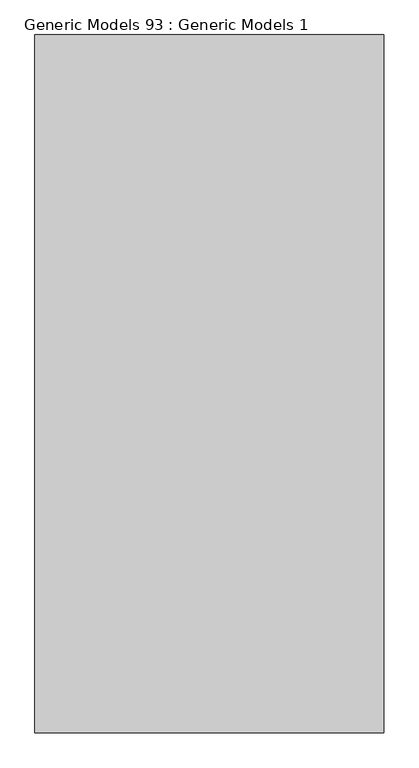
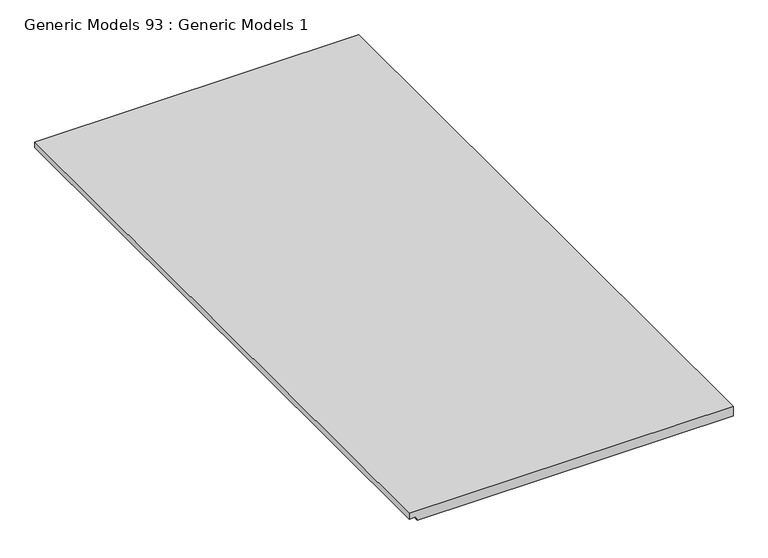
"""IFC4 building model written with IfcOpenShell, lengths in millimetres: proxy geometry, Generic Models 93 : Generic Models 1."""

from ifc_helpers import new_model, si_unit, frame, origin, place, context, project, spatial, polyline, outline, extrude, source, transform, mapped, element, save


def generic_models_93_generic_models_1_4e4062ca(model_context):
    return source(origin(), model_context, "Body", "SweptSolid", [
        extrude(outline(polyline([(2281.1808399, 49813.3451407), (2270.0683399, 49813.3451407), (2270.0683399, 49826.0451407), (2262.1308399, 49828.9341545), (2262.1308399, 50422.9451407), (2281.1808399, 50422.9451407), (2281.1808399, 49813.3451407)])), frame((0.0, 0.0, 0.0), z_axis=(0.0, 1.0, 0.0), x_axis=(0.0, 0.0, 1.0)), (0.0, 0.0, 1.0), 1219.2),
    ])


if __name__ == "__main__":
    model = new_model("IFC4")
    model_context = context("Model", 3, world=origin())
    ifc_project = project(units=[si_unit("LENGTHUNIT", "METRE", prefix="MILLI")], contexts=[model_context])
    site = spatial("IfcSite", under=ifc_project)
    building = spatial("IfcBuilding", under=site)
    placement = place(None, origin())
    generic_models_93_generic_models_1_shape = generic_models_93_generic_models_1_4e4062ca(model_context)
    element("IfcBuildingElementProxy", 1, Name="Generic Models 93 : Generic Models 1", ObjectType="Generic Models 93 : Generic Models 1", at=placement, inside=building, context=model_context, shape_type="MappedRepresentation", body=[
        mapped(generic_models_93_generic_models_1_shape, transform((0.0, 0.0, 0.0), x_axis=(1.0, 0.0, 0.0), y_axis=(0.0, 1.0, 0.0), z_axis=(0.0, 0.0, 1.0))),
    ])
    save(model, "model.ifc")

# Revit data of these elements
# Element 1 (IfcBuildingElementProxy, "Generic Models 93 : Generic Models 1")
#   Materials on its faces: "CEILING AS SCHEDULED"
# Materials
#   "CEILING AS SCHEDULED": class "Generic", colour RGB 255 255 255, transparency 0, Cost = 0
